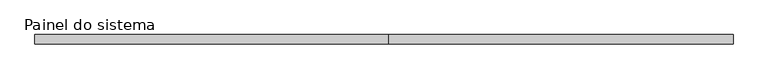
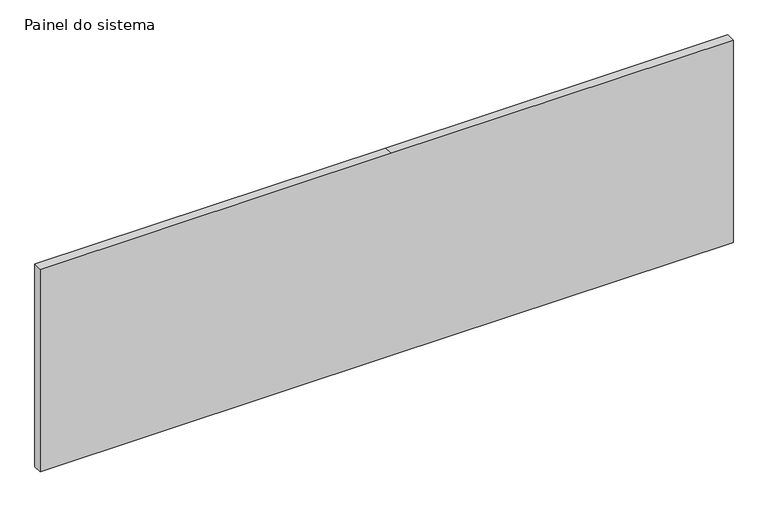
"""IFC4 building model written with IfcOpenShell, lengths in millimetres: plate geometry, Painel do sistema : Envidraçado."""

import ifcopenshell
import ifcopenshell.guid

model = None  # the IFC model being written
_history = None  # IfcOwnerHistory: only IFC2X3 demands one
_inside = {}  # id of a spatial element -> (the spatial element, [elements in it])
_under = {}  # id of a project, library or spatial element -> (it, [spatial elements below it])
_declared = {}  # id of a project -> (the project, [libraries it declares])
_typed = {}  # id of a type object -> (the type object, [elements of that type])
_made_of = {}  # id of a material, layer set ... -> (it, [elements and type objects made of it])


def new_model(schema):
    """Start an empty IFC model of exactly this schema.

    Asked for "IFC4X3", IfcOpenShell would pick the latest addendum, in which some entities
    have other attributes; the version numbers below select the first issue.
    IFC2X3 requires an IfcOwnerHistory on every rooted entity: one is made here for all.
    """
    global model, _history
    if schema == "IFC4X3":
        model = ifcopenshell.file(schema_version=(4, 3, 0, 0))
    else:
        model = ifcopenshell.file(schema=schema)
    _inside.clear()
    _under.clear()
    _declared.clear()
    _typed.clear()
    _made_of.clear()
    _history = None
    if model.schema == "IFC2X3":
        org = make("IfcOrganization", Name="unknown")
        user = make(
            "IfcPersonAndOrganization",
            ThePerson=make("IfcPerson", FamilyName="unknown"),
            TheOrganization=org,
        )
        app = make(
            "IfcApplication",
            ApplicationDeveloper=org,
            Version="unknown",
            ApplicationFullName="unknown",
            ApplicationIdentifier="unknown",
        )
        _history = make(
            "IfcOwnerHistory",
            OwningUser=user,
            OwningApplication=app,
            ChangeAction="ADDED",
            CreationDate=0,
        )
    return model


def make(cls, **values):
    """One entity of the class cls with the attributes given. An attribute that is None is left unset."""
    return model.create_entity(
        cls, **{name: value for name, value in values.items() if value is not None}
    )


def rooted(cls, **values):
    """An entity with a GlobalId (a new one), such as an element, a storey or a relation."""
    return make(cls, GlobalId=ifcopenshell.guid.new(), OwnerHistory=_history, **values)


def si_unit(unit_type, name, prefix=None):
    """IfcSIUnit, for example si_unit("LENGTHUNIT", "METRE", prefix="MILLI")."""
    return make("IfcSIUnit", UnitType=unit_type, Prefix=prefix, Name=name)


def assignment(units):
    """IfcUnitAssignment: the units of a project."""
    return None if units is None else make("IfcUnitAssignment", Units=units)


def point(xyz):
    """IfcCartesianPoint."""
    return None if xyz is None else make("IfcCartesianPoint", Coordinates=xyz)


def direction(xyz):
    """IfcDirection."""
    return None if xyz is None else make("IfcDirection", DirectionRatios=xyz)


def frame(location, z_axis=None, x_axis=None):
    """IfcAxis2Placement3D, a coordinate frame: its origin and axes. An axis left out is left unset."""
    return make(
        "IfcAxis2Placement3D",
        Location=point(location),
        Axis=direction(z_axis),
        RefDirection=direction(x_axis),
    )


def origin():
    """The frame at (0, 0, 0) with its axes left unset."""
    return frame((0.0, 0.0, 0.0))


def place(relative_to, where):
    """IfcLocalPlacement: puts the frame where relative to a parent placement (None: the world)."""
    return make(
        "IfcLocalPlacement", PlacementRelTo=relative_to, RelativePlacement=where
    )


def context(
    kind, dimensions, precision=None, world=None, true_north=None, identifier=None
):
    """IfcGeometricRepresentationContext, for example the 3D "Model" context."""
    return make(
        "IfcGeometricRepresentationContext",
        ContextIdentifier=identifier,
        ContextType=kind,
        CoordinateSpaceDimension=dimensions,
        Precision=precision,
        WorldCoordinateSystem=world,
        TrueNorth=true_north,
    )


def project(units=None, contexts=None):
    """IfcProject with its units and contexts."""
    return rooted(
        "IfcProject",
        Name="project",
        RepresentationContexts=contexts,
        UnitsInContext=assignment(units),
    )


def spatial(cls, under=None, at=None, **own):
    """A site, building, storey or space (cls), placed at a placement, below another one or the project."""
    s = rooted(cls, ObjectPlacement=at, **own)
    if under is not None:
        _under.setdefault(under.id(), (under, []))[1].append(s)
    return s


def polyline(points):
    """IfcPolyline through the points."""
    return make("IfcPolyline", Points=[point(p) for p in points])


def outline(outer, holes=None, kind="AREA"):
    """IfcArbitraryClosedProfileDef: a profile drawn as a closed curve; with holes, ...WithVoids."""
    if holes is None:
        return make("IfcArbitraryClosedProfileDef", ProfileType=kind, OuterCurve=outer)
    return make(
        "IfcArbitraryProfileDefWithVoids",
        ProfileType=kind,
        OuterCurve=outer,
        InnerCurves=holes,
    )


def extrude(swept, where, along, depth):
    """IfcExtrudedAreaSolid: the profile swept, set in the frame where, extruded along a direction by depth."""
    return make(
        "IfcExtrudedAreaSolid",
        SweptArea=swept,
        Position=where,
        ExtrudedDirection=direction(along),
        Depth=depth,
    )


def shape(context_of_items, identifier, shape_type, items):
    """IfcShapeRepresentation: the items that make up one representation, for example the "Body"."""
    return make(
        "IfcShapeRepresentation",
        ContextOfItems=context_of_items,
        RepresentationIdentifier=identifier,
        RepresentationType=shape_type,
        Items=items,
    )


def source(mapping_origin, context_of_items, identifier, shape_type, items):
    """IfcRepresentationMap: a shape defined once, which mapped items show again and again."""
    return make(
        "IfcRepresentationMap",
        MappingOrigin=mapping_origin,
        MappedRepresentation=shape(context_of_items, identifier, shape_type, items),
    )


def transform(
    local_origin,
    x_axis=None,
    y_axis=None,
    z_axis=None,
    scale=None,
    scale2=None,
    scale3=None,
    uniform=True,
):
    """IfcCartesianTransformationOperator3D, or its non-uniform kind. x_axis, y_axis, z_axis: its Axis1, 2, 3."""
    if uniform:
        return make(
            "IfcCartesianTransformationOperator3D",
            Axis1=direction(x_axis),
            Axis2=direction(y_axis),
            LocalOrigin=point(local_origin),
            Scale=scale,
            Axis3=direction(z_axis),
        )
    return make(
        "IfcCartesianTransformationOperator3DnonUniform",
        Axis1=direction(x_axis),
        Axis2=direction(y_axis),
        LocalOrigin=point(local_origin),
        Scale=scale,
        Axis3=direction(z_axis),
        Scale2=scale2,
        Scale3=scale3,
    )


def mapped(mapping_source, mapping_target):
    """IfcMappedItem: shows the shape of a source again, moved by a transform."""
    return make(
        "IfcMappedItem", MappingSource=mapping_source, MappingTarget=mapping_target
    )


def made_of(thing, what):
    """Note that an element or type object is made of a material, layer set ...; save() writes the relation."""
    if what is not None:
        _made_of.setdefault(what.id(), (what, []))[1].append(thing)
    return thing


def element(
    cls,
    number,
    at=None,
    inside=None,
    cuts=None,
    type_object=None,
    material=None,
    context=None,
    identifier="Body",
    shape_type=None,
    held_by="IfcProductDefinitionShape",
    body=None,
    shapes=None,
    **own,
):
    """One element of the class cls, such as IfcWall. Its Tag is "e" and its number.

    at: its placement. inside: the storey or other place that contains it. cuts: it is an
    opening in that element (IfcRelVoidsElement). A single representation is given by context,
    identifier, shape_type and body (its items); several are given by shapes. held_by: the class
    of the entity that holds the representations. save() writes the other relations.
    """
    e = rooted(cls, Tag="e%d" % number, ObjectPlacement=at, **own)
    if body is not None:
        shapes = [shape(context, identifier, shape_type, body)]
    if shapes is not None:
        e.Representation = make(held_by, Representations=shapes)
    if inside is not None:
        _inside.setdefault(inside.id(), (inside, []))[1].append(e)
    if cuts is not None:
        rooted(
            "IfcRelVoidsElement", RelatingBuildingElement=cuts, RelatedOpeningElement=e
        )
    if type_object is not None:
        _typed.setdefault(type_object.id(), (type_object, []))[1].append(e)
    return made_of(e, material)


def aggregate(whole, parts):
    """IfcRelAggregates: a whole, such as a stair, and the parts it consists of."""
    return rooted("IfcRelAggregates", RelatingObject=whole, RelatedObjects=parts)


def save(model, path):
    """Write the relations noted so far, then the file.

    IfcRelAggregates (storeys below a building ...), IfcRelContainedInSpatialStructure (elements
    in a storey), IfcRelDefinesByType, IfcRelAssociatesMaterial and IfcRelDeclares: one each for
    every whole, place, type object, material and project.
    """
    for whole, parts in _under.values():
        aggregate(whole, parts)
    for where, things in _inside.values():
        rooted(
            "IfcRelContainedInSpatialStructure",
            RelatedElements=things,
            RelatingStructure=where,
        )
    for kind, things in _typed.values():
        rooted("IfcRelDefinesByType", RelatedObjects=things, RelatingType=kind)
    for what, things in _made_of.values():
        rooted("IfcRelAssociatesMaterial", RelatedObjects=things, RelatingMaterial=what)
    for by, libraries in _declared.values():
        rooted("IfcRelDeclares", RelatingContext=by, RelatedDefinitions=libraries)
    model.write(path)


def painel_do_sistema_1f2b63a2(model_context):
    return source(origin(), model_context, "Body", "SweptSolid", [
        extrude(outline(polyline([(0.0, -954.2100001), (0.0, 12.4999998), (0.0, 954.2100001), (590.0, 954.2100001), (590.0, 12.4999998), (590.0, -954.2100001), (0.0, -954.2100001)])), frame((0.0, -49.5, 0.0), z_axis=(0.0, 1.0, 0.0), x_axis=(0.0, 0.0, 1.0)), (0.0, 0.0, 1.0), 25.0),
    ])


if __name__ == "__main__":
    model = new_model("IFC4")
    model_context = context("Model", 3, world=origin())
    ifc_project = project(units=[si_unit("LENGTHUNIT", "METRE", prefix="MILLI")], contexts=[model_context])
    site = spatial("IfcSite", under=ifc_project)
    building = spatial("IfcBuilding", under=site)
    placement = place(None, origin())
    painel_do_sistema_shape = painel_do_sistema_1f2b63a2(model_context)
    element("IfcPlate", 1, ObjectType="Painel do sistema : Envidraçado", at=placement, inside=building, context=model_context, shape_type="MappedRepresentation", body=[
        mapped(painel_do_sistema_shape, transform((0.0, 0.0, 0.0), x_axis=(1.0, 0.0, 0.0), y_axis=(0.0, 1.0, 0.0), z_axis=(0.0, 0.0, 1.0))),
    ])
    save(model, "model.ifc")

# Revit data of these elements
# Type "Painel do sistema : Envidraçado"
#   Construction Type Id = "GSP4R"
#   Analytic Construction = "Vidraça única Pilkington 1/8 pol"
#   Visual Light Transmittance = 0.9
#   Solar Heat Gain Coefficient = 0.86
#   Heat Transfer Coefficient (U) = 6.7069 W/(m²·K)
# Element 1 (IfcPlate, "Painel do sistema : Envidraçado")
#   Materials on its faces: ".VIDRO GENÉRICO"
# Materials
#   ".VIDRO GENÉRICO": class ".CC_VIDRO", colour RGB 0 128 192, transparency 0.9, Description = "Vidro comum", Cost = 0
